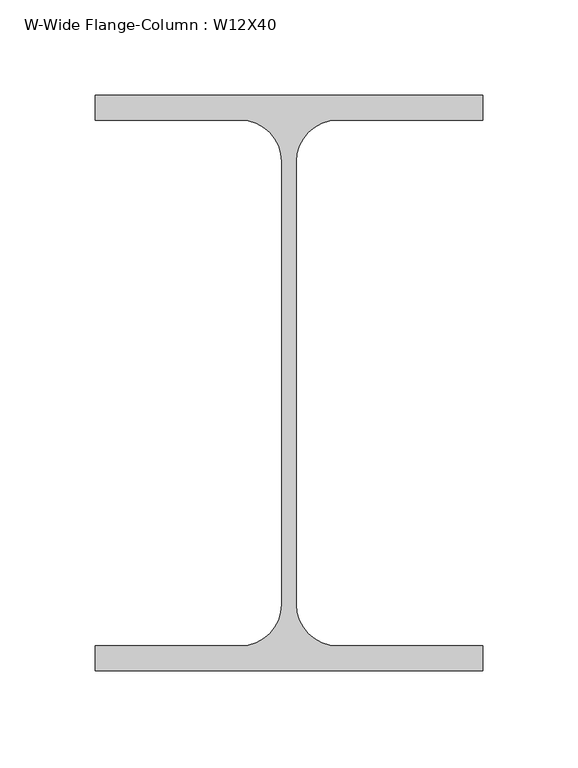
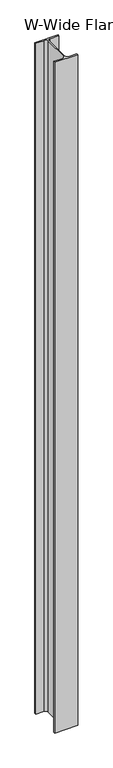
"""IFC4 building model written with IfcOpenShell, lengths in millimetres: column geometry, W-Wide Flange-Column : W12X40."""

import ifcopenshell
import ifcopenshell.guid

model = None  # the IFC model being written
_history = None  # IfcOwnerHistory: only IFC2X3 demands one
_inside = {}  # id of a spatial element -> (the spatial element, [elements in it])
_under = {}  # id of a project, library or spatial element -> (it, [spatial elements below it])
_declared = {}  # id of a project -> (the project, [libraries it declares])
_typed = {}  # id of a type object -> (the type object, [elements of that type])
_made_of = {}  # id of a material, layer set ... -> (it, [elements and type objects made of it])


def new_model(schema):
    """Start an empty IFC model of exactly this schema.

    Asked for "IFC4X3", IfcOpenShell would pick the latest addendum, in which some entities
    have other attributes; the version numbers below select the first issue.
    IFC2X3 requires an IfcOwnerHistory on every rooted entity: one is made here for all.
    """
    global model, _history
    if schema == "IFC4X3":
        model = ifcopenshell.file(schema_version=(4, 3, 0, 0))
    else:
        model = ifcopenshell.file(schema=schema)
    _inside.clear()
    _under.clear()
    _declared.clear()
    _typed.clear()
    _made_of.clear()
    _history = None
    if model.schema == "IFC2X3":
        org = make("IfcOrganization", Name="unknown")
        user = make(
            "IfcPersonAndOrganization",
            ThePerson=make("IfcPerson", FamilyName="unknown"),
            TheOrganization=org,
        )
        app = make(
            "IfcApplication",
            ApplicationDeveloper=org,
            Version="unknown",
            ApplicationFullName="unknown",
            ApplicationIdentifier="unknown",
        )
        _history = make(
            "IfcOwnerHistory",
            OwningUser=user,
            OwningApplication=app,
            ChangeAction="ADDED",
            CreationDate=0,
        )
    return model


def make(cls, **values):
    """One entity of the class cls with the attributes given. An attribute that is None is left unset."""
    return model.create_entity(
        cls, **{name: value for name, value in values.items() if value is not None}
    )


def rooted(cls, **values):
    """An entity with a GlobalId (a new one), such as an element, a storey or a relation."""
    return make(cls, GlobalId=ifcopenshell.guid.new(), OwnerHistory=_history, **values)


def si_unit(unit_type, name, prefix=None):
    """IfcSIUnit, for example si_unit("LENGTHUNIT", "METRE", prefix="MILLI")."""
    return make("IfcSIUnit", UnitType=unit_type, Prefix=prefix, Name=name)


def assignment(units):
    """IfcUnitAssignment: the units of a project."""
    return None if units is None else make("IfcUnitAssignment", Units=units)


def point(xyz):
    """IfcCartesianPoint."""
    return None if xyz is None else make("IfcCartesianPoint", Coordinates=xyz)


def direction(xyz):
    """IfcDirection."""
    return None if xyz is None else make("IfcDirection", DirectionRatios=xyz)


def frame(location, z_axis=None, x_axis=None):
    """IfcAxis2Placement3D, a coordinate frame: its origin and axes. An axis left out is left unset."""
    return make(
        "IfcAxis2Placement3D",
        Location=point(location),
        Axis=direction(z_axis),
        RefDirection=direction(x_axis),
    )


def frame_2d(location, x_axis=None):
    """IfcAxis2Placement2D, a coordinate frame in the plane: its origin and x axis."""
    return make(
        "IfcAxis2Placement2D", Location=point(location), RefDirection=direction(x_axis)
    )


def origin():
    """The frame at (0, 0, 0) with its axes left unset."""
    return frame((0.0, 0.0, 0.0))


def place(relative_to, where):
    """IfcLocalPlacement: puts the frame where relative to a parent placement (None: the world)."""
    return make(
        "IfcLocalPlacement", PlacementRelTo=relative_to, RelativePlacement=where
    )


def context(
    kind, dimensions, precision=None, world=None, true_north=None, identifier=None
):
    """IfcGeometricRepresentationContext, for example the 3D "Model" context."""
    return make(
        "IfcGeometricRepresentationContext",
        ContextIdentifier=identifier,
        ContextType=kind,
        CoordinateSpaceDimension=dimensions,
        Precision=precision,
        WorldCoordinateSystem=world,
        TrueNorth=true_north,
    )


def project(units=None, contexts=None):
    """IfcProject with its units and contexts."""
    return rooted(
        "IfcProject",
        Name="project",
        RepresentationContexts=contexts,
        UnitsInContext=assignment(units),
    )


def spatial(cls, under=None, at=None, **own):
    """A site, building, storey or space (cls), placed at a placement, below another one or the project."""
    s = rooted(cls, ObjectPlacement=at, **own)
    if under is not None:
        _under.setdefault(under.id(), (under, []))[1].append(s)
    return s


def polyline(points):
    """IfcPolyline through the points."""
    return make("IfcPolyline", Points=[point(p) for p in points])


def circle_curve(where, radius):
    """IfcCircle in the frame where."""
    return make("IfcCircle", Position=where, Radius=radius)


def trimmed(basis, trim1, trim2, sense, master):
    """IfcTrimmedCurve: the piece of a basis curve between two trims."""
    return make(
        "IfcTrimmedCurve",
        BasisCurve=basis,
        Trim1=trim1,
        Trim2=trim2,
        SenseAgreement=sense,
        MasterRepresentation=master,
    )


def segment(curve, same_sense, transition):
    """IfcCompositeCurveSegment."""
    return make(
        "IfcCompositeCurveSegment",
        Transition=transition,
        SameSense=same_sense,
        ParentCurve=curve,
    )


def composite_curve(segments, self_intersect=None):
    """IfcCompositeCurve: segments joined end to end."""
    return make("IfcCompositeCurve", Segments=segments, SelfIntersect=self_intersect)


def outline(outer, holes=None, kind="AREA"):
    """IfcArbitraryClosedProfileDef: a profile drawn as a closed curve; with holes, ...WithVoids."""
    if holes is None:
        return make("IfcArbitraryClosedProfileDef", ProfileType=kind, OuterCurve=outer)
    return make(
        "IfcArbitraryProfileDefWithVoids",
        ProfileType=kind,
        OuterCurve=outer,
        InnerCurves=holes,
    )


def extrude(swept, where, along, depth):
    """IfcExtrudedAreaSolid: the profile swept, set in the frame where, extruded along a direction by depth."""
    return make(
        "IfcExtrudedAreaSolid",
        SweptArea=swept,
        Position=where,
        ExtrudedDirection=direction(along),
        Depth=depth,
    )


def shape(context_of_items, identifier, shape_type, items):
    """IfcShapeRepresentation: the items that make up one representation, for example the "Body"."""
    return make(
        "IfcShapeRepresentation",
        ContextOfItems=context_of_items,
        RepresentationIdentifier=identifier,
        RepresentationType=shape_type,
        Items=items,
    )


def source(mapping_origin, context_of_items, identifier, shape_type, items):
    """IfcRepresentationMap: a shape defined once, which mapped items show again and again."""
    return make(
        "IfcRepresentationMap",
        MappingOrigin=mapping_origin,
        MappedRepresentation=shape(context_of_items, identifier, shape_type, items),
    )


def transform(
    local_origin,
    x_axis=None,
    y_axis=None,
    z_axis=None,
    scale=None,
    scale2=None,
    scale3=None,
    uniform=True,
):
    """IfcCartesianTransformationOperator3D, or its non-uniform kind. x_axis, y_axis, z_axis: its Axis1, 2, 3."""
    if uniform:
        return make(
            "IfcCartesianTransformationOperator3D",
            Axis1=direction(x_axis),
            Axis2=direction(y_axis),
            LocalOrigin=point(local_origin),
            Scale=scale,
            Axis3=direction(z_axis),
        )
    return make(
        "IfcCartesianTransformationOperator3DnonUniform",
        Axis1=direction(x_axis),
        Axis2=direction(y_axis),
        LocalOrigin=point(local_origin),
        Scale=scale,
        Axis3=direction(z_axis),
        Scale2=scale2,
        Scale3=scale3,
    )


def mapped(mapping_source, mapping_target):
    """IfcMappedItem: shows the shape of a source again, moved by a transform."""
    return make(
        "IfcMappedItem", MappingSource=mapping_source, MappingTarget=mapping_target
    )


def made_of(thing, what):
    """Note that an element or type object is made of a material, layer set ...; save() writes the relation."""
    if what is not None:
        _made_of.setdefault(what.id(), (what, []))[1].append(thing)
    return thing


def element(
    cls,
    number,
    at=None,
    inside=None,
    cuts=None,
    type_object=None,
    material=None,
    context=None,
    identifier="Body",
    shape_type=None,
    held_by="IfcProductDefinitionShape",
    body=None,
    shapes=None,
    **own,
):
    """One element of the class cls, such as IfcWall. Its Tag is "e" and its number.

    at: its placement. inside: the storey or other place that contains it. cuts: it is an
    opening in that element (IfcRelVoidsElement). A single representation is given by context,
    identifier, shape_type and body (its items); several are given by shapes. held_by: the class
    of the entity that holds the representations. save() writes the other relations.
    """
    e = rooted(cls, Tag="e%d" % number, ObjectPlacement=at, **own)
    if body is not None:
        shapes = [shape(context, identifier, shape_type, body)]
    if shapes is not None:
        e.Representation = make(held_by, Representations=shapes)
    if inside is not None:
        _inside.setdefault(inside.id(), (inside, []))[1].append(e)
    if cuts is not None:
        rooted(
            "IfcRelVoidsElement", RelatingBuildingElement=cuts, RelatedOpeningElement=e
        )
    if type_object is not None:
        _typed.setdefault(type_object.id(), (type_object, []))[1].append(e)
    return made_of(e, material)


def aggregate(whole, parts):
    """IfcRelAggregates: a whole, such as a stair, and the parts it consists of."""
    return rooted("IfcRelAggregates", RelatingObject=whole, RelatedObjects=parts)


def save(model, path):
    """Write the relations noted so far, then the file.

    IfcRelAggregates (storeys below a building ...), IfcRelContainedInSpatialStructure (elements
    in a storey), IfcRelDefinesByType, IfcRelAssociatesMaterial and IfcRelDeclares: one each for
    every whole, place, type object, material and project.
    """
    for whole, parts in _under.values():
        aggregate(whole, parts)
    for where, things in _inside.values():
        rooted(
            "IfcRelContainedInSpatialStructure",
            RelatedElements=things,
            RelatingStructure=where,
        )
    for kind, things in _typed.values():
        rooted("IfcRelDefinesByType", RelatedObjects=things, RelatingType=kind)
    for what, things in _made_of.values():
        rooted("IfcRelAssociatesMaterial", RelatedObjects=things, RelatingMaterial=what)
    for by, libraries in _declared.values():
        rooted("IfcRelDeclares", RelatingContext=by, RelatedDefinitions=libraries)
    model.write(path)


def w_wide_flange_column_w12x40_573c2af4(model_context):
    return source(origin(), model_context, "Body", "SweptSolid", [
        extrude(outline(composite_curve([segment(polyline([(101.727, 151.13), (101.727, 138.049), (25.5905, 138.049)]), True, "CONTINUOUS"), segment(trimmed(circle_curve(frame_2d((25.5905, 116.205)), 21.844), [point((25.5905, 138.049))], [point((3.7465, 116.205))], True, "CARTESIAN"), True, "CONTINUOUS"), segment(polyline([(3.7465, 116.205), (3.7465, -116.205)]), True, "CONTINUOUS"), segment(trimmed(circle_curve(frame_2d((25.5905, -116.205)), 21.844), [point((3.7465, -116.205))], [point((25.5905, -138.049))], True, "CARTESIAN"), True, "CONTINUOUS"), segment(polyline([(25.5905, -138.049), (101.727, -138.049), (101.727, -151.13), (-101.727, -151.13), (-101.727, -138.049), (-25.5905, -138.049)]), True, "CONTINUOUS"), segment(trimmed(circle_curve(frame_2d((-25.5905, -116.205)), 21.844), [point((-25.5905, -138.049))], [point((-3.7465, -116.205))], True, "CARTESIAN"), True, "CONTINUOUS"), segment(polyline([(-3.7465, -116.205), (-3.7465, 116.205)]), True, "CONTINUOUS"), segment(trimmed(circle_curve(frame_2d((-25.5905, 116.205)), 21.844), [point((-3.7465, 116.205))], [point((-25.5905, 138.049))], True, "CARTESIAN"), True, "CONTINUOUS"), segment(polyline([(-25.5905, 138.049), (-101.727, 138.049), (-101.727, 151.13), (101.727, 151.13)]), True, "CONTINUOUS")], self_intersect=False)), frame((0.0, 0.0, 23317.2), z_axis=(0.0, 0.0, 1.0), x_axis=(1.0, 0.0, 0.0)), (0.0, 0.0, 1.0), 6248.4),
    ])


if __name__ == "__main__":
    model = new_model("IFC4")
    model_context = context("Model", 3, world=origin())
    ifc_project = project(units=[si_unit("LENGTHUNIT", "METRE", prefix="MILLI")], contexts=[model_context])
    site = spatial("IfcSite", under=ifc_project)
    building = spatial("IfcBuilding", under=site)
    placement = place(None, origin())
    w_wide_flange_column_w12x40_shape = w_wide_flange_column_w12x40_573c2af4(model_context)
    element("IfcColumn", 1, ObjectType="W-Wide Flange-Column : W12X40", at=placement, inside=building, context=model_context, shape_type="MappedRepresentation", body=[
        mapped(w_wide_flange_column_w12x40_shape, transform((0.0, 0.0, 0.0), x_axis=(1.0, 0.0, 0.0), y_axis=(0.0, 1.0, 0.0), z_axis=(0.0, 0.0, 1.0))),
    ])
    save(model, "model.ifc")

# Revit data of these elements
# Type "W-Wide Flange-Column : W12X40"
#   Assembly Code = "B10"
#   W = 40
#   bf = 0' - 8.01"
#   d = 0' - 11.9"
#   k = 0' - 1 3/8"
#   kr = 0' - 0.86"
#   tf = 0' - 0.515"
#   tw = 0' - 0.295"
#   A = 0.08125 SF
#   Structural Material [instance default] = Steel ASTM A992
# Element 1 (IfcColumn, "W-Wide Flange-Column : W12X40")
#   Materials on its faces: "Steel ASTM A992"
# Materials
#   "Steel ASTM A992": class "Metal", colour RGB 199 199 199, transparency 0, Description = "Structural steel 50ksi", Cost = 0
